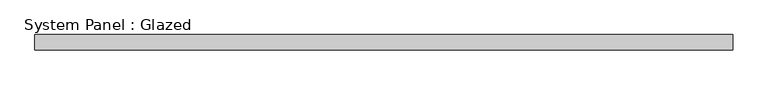
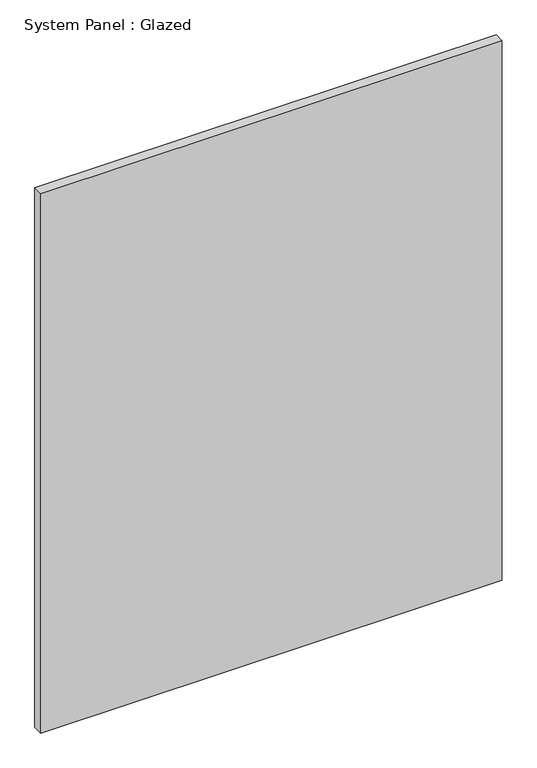
"""IFC4 building model written with IfcOpenShell, lengths in millimetres: plate geometry, System Panel : Glazed."""

from ifc_helpers import new_model, si_unit, origin, origin_with_axes, place, context, project, spatial, polyline, outline, extrude, source, transform, mapped, element, save


def system_panel_glazed_b81d08ea(model_context):
    return source(origin(), model_context, "Body", "SweptSolid", [
        extrude(outline(polyline([(566.6666667, 24.5), (-566.6666667, 24.5), (-566.6666667, 49.5), (566.6666667, 49.5), (566.6666667, 24.5)])), origin_with_axes(), (0.0, 0.0, 1.0), 1400.0),
    ])


if __name__ == "__main__":
    model = new_model("IFC4")
    model_context = context("Model", 3, world=origin())
    ifc_project = project(units=[si_unit("LENGTHUNIT", "METRE", prefix="MILLI")], contexts=[model_context])
    site = spatial("IfcSite", under=ifc_project)
    building = spatial("IfcBuilding", under=site)
    placement = place(None, origin())
    system_panel_glazed_shape = system_panel_glazed_b81d08ea(model_context)
    element("IfcPlate", 1, ObjectType="System Panel : Glazed", at=placement, inside=building, context=model_context, shape_type="MappedRepresentation", body=[
        mapped(system_panel_glazed_shape, transform((0.0, 0.0, 0.0), x_axis=(1.0, 0.0, 0.0), y_axis=(0.0, 1.0, 0.0), z_axis=(0.0, 0.0, 1.0))),
    ])
    save(model, "model.ifc")

# Revit data of these elements
# Element 1 (IfcPlate, "System Panel : Glazed")
#   Materials on its faces: "Glass"
# Materials
#   "Glass": class "Glass", colour RGB 0 128 192, transparency 0.9
